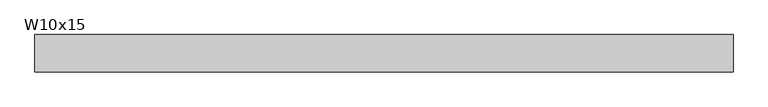
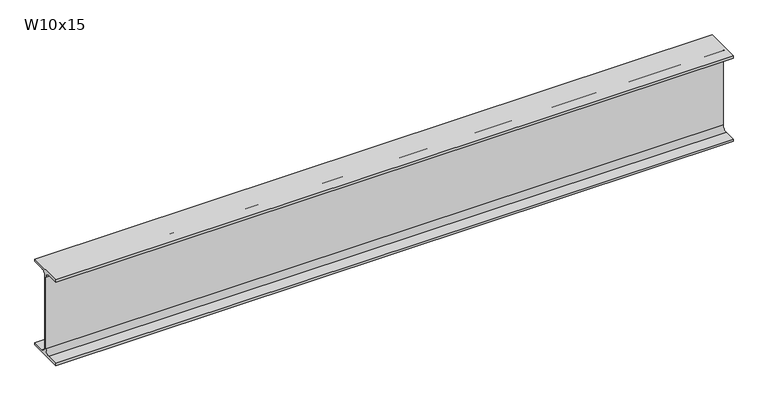
"""IFC4 building model written with IfcOpenShell, lengths in millimetres: beam geometry, RME W-Wide Flange : W10x15."""

from ifc_helpers import new_model, si_unit, point, frame, frame_2d, origin, place, context, project, spatial, polyline, circle_curve, trimmed, segment, composite_curve, outline, extrude, source, transform, mapped, element, save


def w10x15_b22fd661(model_context):
    return source(origin(), model_context, "Body", "SweptSolid", [
        extrude(outline(composite_curve([segment(polyline([(50.8, -120.142), (50.8, -127.0), (-50.8, -127.0), (-50.8, -120.142), (-16.7005, -120.142)]), True, "CONTINUOUS"), segment(trimmed(circle_curve(frame_2d((-16.7005, -106.3625)), 13.7795), [point((-16.7005, -120.142))], [point((-2.921, -106.3625))], True, "CARTESIAN"), True, "CONTINUOUS"), segment(polyline([(-2.921, -106.3625), (-2.921, 106.3625)]), True, "CONTINUOUS"), segment(trimmed(circle_curve(frame_2d((-16.7005, 106.3625)), 13.7795), [point((-2.921, 106.3625))], [point((-16.7005, 120.142))], True, "CARTESIAN"), True, "CONTINUOUS"), segment(polyline([(-16.7005, 120.142), (-50.8, 120.142), (-50.8, 127.0), (50.8, 127.0), (50.8, 120.142), (16.7005, 120.142)]), True, "CONTINUOUS"), segment(trimmed(circle_curve(frame_2d((16.7005, 106.3625)), 13.7795), [point((16.7005, 120.142))], [point((2.921, 106.3625))], True, "CARTESIAN"), True, "CONTINUOUS"), segment(polyline([(2.921, 106.3625), (2.921, -106.3625)]), True, "CONTINUOUS"), segment(trimmed(circle_curve(frame_2d((16.7005, -106.3625)), 13.7795), [point((2.921, -106.3625))], [point((16.7005, -120.142))], True, "CARTESIAN"), True, "CONTINUOUS"), segment(polyline([(16.7005, -120.142), (50.8, -120.142)]), True, "CONTINUOUS")], self_intersect=False)), frame((-1091.893007, 0.0, 0.0), z_axis=(1.0, 0.0, 0.0), x_axis=(0.0, 1.0, 0.0)), (0.0, 0.0, 1.0), 1897.1920058),
    ])


if __name__ == "__main__":
    model = new_model("IFC4")
    model_context = context("Model", 3, world=origin())
    ifc_project = project(units=[si_unit("LENGTHUNIT", "METRE", prefix="MILLI")], contexts=[model_context])
    site = spatial("IfcSite", under=ifc_project)
    building = spatial("IfcBuilding", under=site)
    placement = place(None, origin())
    w10x15_shape = w10x15_b22fd661(model_context)
    element("IfcBeam", 1, ObjectType="RME W-Wide Flange : W10x15", at=placement, inside=building, context=model_context, shape_type="MappedRepresentation", body=[
        mapped(w10x15_shape, transform((0.0, 0.0, 0.0), x_axis=(1.0, 0.0, 0.0), y_axis=(0.0, 1.0, 0.0), z_axis=(0.0, 0.0, 1.0))),
    ])
    save(model, "model.ifc")

# Revit data of these elements
# Type "RME W-Wide Flange : W10x15"
#   WELD P [instance default] = ""
#   WELD LE [instance default] = ""
#   WELD D [instance default] = ""
#   TOP SECTION SIZE [instance default] = ""
#   TOP SECTION LENGTH [instance default] = ""
#   REMARKS [instance default] = ""
#   REINF TYPE [instance default] = ""
#   Nominal Size = "W24"
#   End Bearing Capacity [instance default] = ""
#   BOT SECTION SIZE [instance default] = ""
#   BOT SECTION LENGTH [instance default] = ""
#   Assembly Code = "B10"
#   W = 15
#   Start Extension Calculation [instance default] = 10' - 0"
#   Start Extension [instance default] = -0' - 0 1/2"
#   End Extension Calculation [instance default] = 10' - 0"
#   End Extension [instance default] = -0' - 0 1/2"
#   Length [instance default] = 5' - 0"
#   bf = 0' - 4"
#   d = 0' - 10"
#   k = 0' - 0 13/16"
#   k2 = 0' - 0.5425"
#   tf = 0' - 0.27"
#   tw = 0' - 0.23"
#   A = 0.030625 SF
#   Structural Material [instance default] = Metal - Steel - ASTM A992
# Element 1 (IfcBeam, "RME W-Wide Flange : W10x15")
#   Start Extension Calculation = 11' - 5.90162"
#   Start Extension = 1' - 5.40162"
#   Length = 5' - 9"
#   Materials on its faces: "Metal - Steel - ASTM A992"
# Materials
#   "Metal - Steel - ASTM A992": class "Metal", colour RGB 255 128 0, transparency 0
